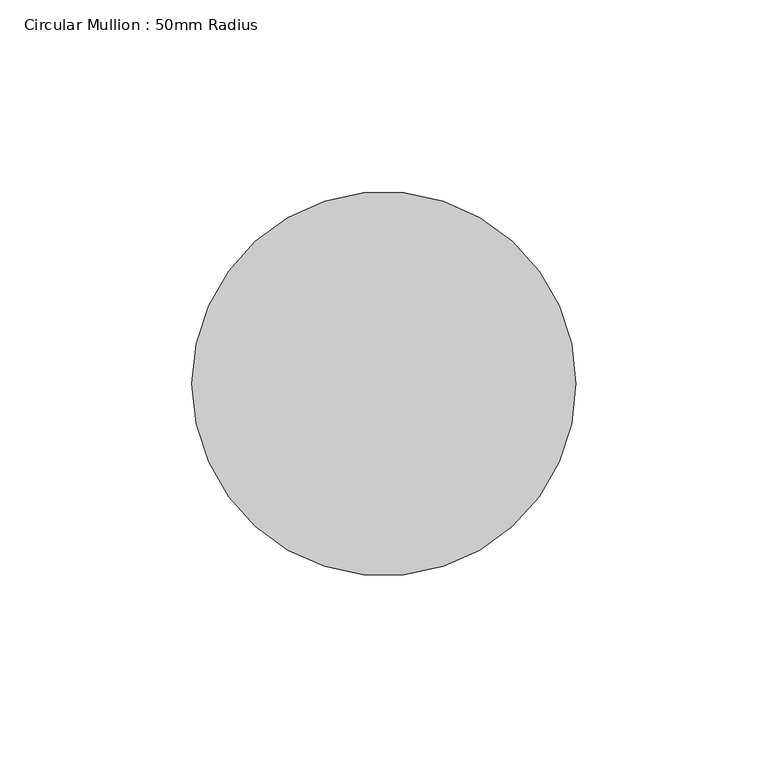
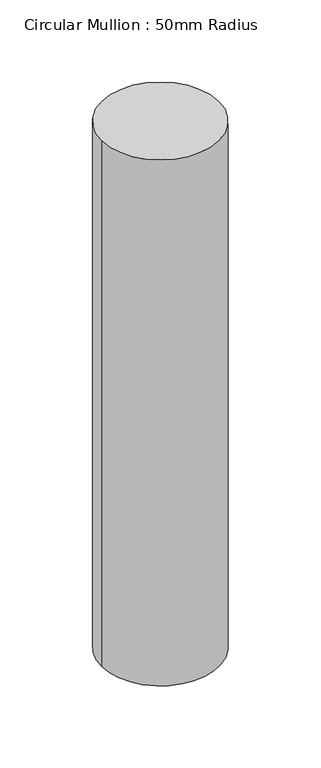
"""IFC4 building model written with IfcOpenShell, lengths in millimetres: member geometry, Circular Mullion : 50mm Radius."""

from ifc_helpers import new_model, si_unit, point, frame, origin, origin_2d, place, context, project, spatial, circle_curve, trimmed, segment, composite_curve, outline, extrude, source, transform, mapped, element, save


def circular_mullion_50mm_radius_95129a9f(model_context):
    return source(origin(), model_context, "Body", "SweptSolid", [
        extrude(outline(composite_curve([segment(trimmed(circle_curve(origin_2d(), 50.0), [point((50.0, 0.0))], [point((-50.0, 0.0))], False, "CARTESIAN"), True, "CONTINUOUS"), segment(trimmed(circle_curve(origin_2d(), 50.0), [point((-50.0, 0.0))], [point((50.0, 0.0))], False, "CARTESIAN"), True, "CONTINUOUS")], self_intersect=False)), frame((0.0, 0.0, -473.2843109), z_axis=(0.0, 0.0, 1.0), x_axis=(1.0, 0.0, 0.0)), (0.0, 0.0, 1.0), 473.2843109),
    ])


if __name__ == "__main__":
    model = new_model("IFC4")
    model_context = context("Model", 3, world=origin())
    ifc_project = project(units=[si_unit("LENGTHUNIT", "METRE", prefix="MILLI")], contexts=[model_context])
    site = spatial("IfcSite", under=ifc_project)
    building = spatial("IfcBuilding", under=site)
    placement = place(None, origin())
    circular_mullion_50mm_radius_shape = circular_mullion_50mm_radius_95129a9f(model_context)
    element("IfcMember", 1, ObjectType="Circular Mullion : 50mm Radius", at=placement, inside=building, context=model_context, shape_type="MappedRepresentation", body=[
        mapped(circular_mullion_50mm_radius_shape, transform((0.0, 0.0, 0.0), x_axis=(1.0, 0.0, 0.0), y_axis=(0.0, 1.0, 0.0), z_axis=(0.0, 0.0, 1.0))),
    ])
    save(model, "model.ifc")

# Revit data of these elements
# Type "Circular Mullion : 50mm Radius"
#   built-in parameter 1007350 = 0.164042 (stored number, unit not read)
# Element 1 (IfcMember, "Circular Mullion : 50mm Radius")
#   Materials on its faces: "Aluminium"
# Materials
#   "Aluminium": class "Metal", colour RGB 247 247 247, transparency 0, Description = "Aluminium 6061", Cost = 0
